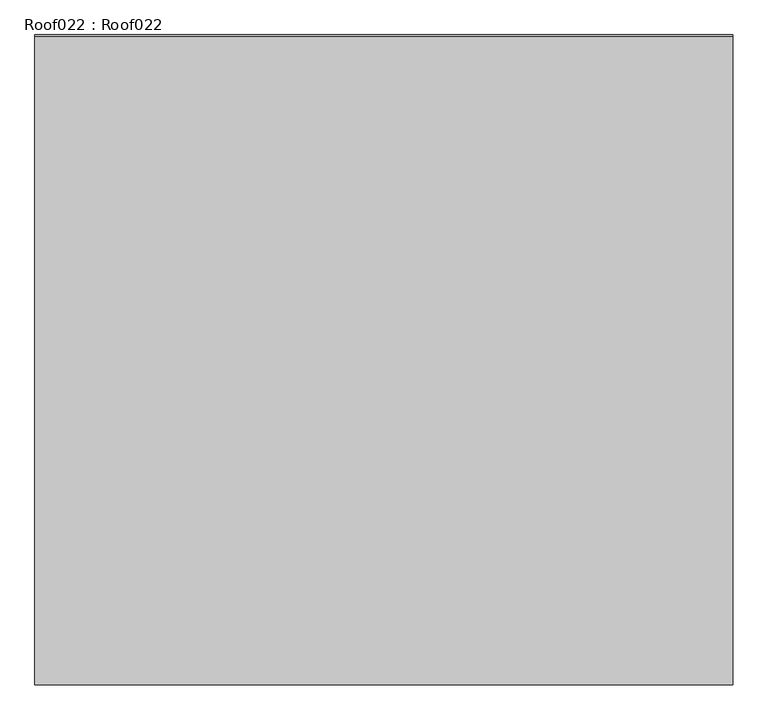
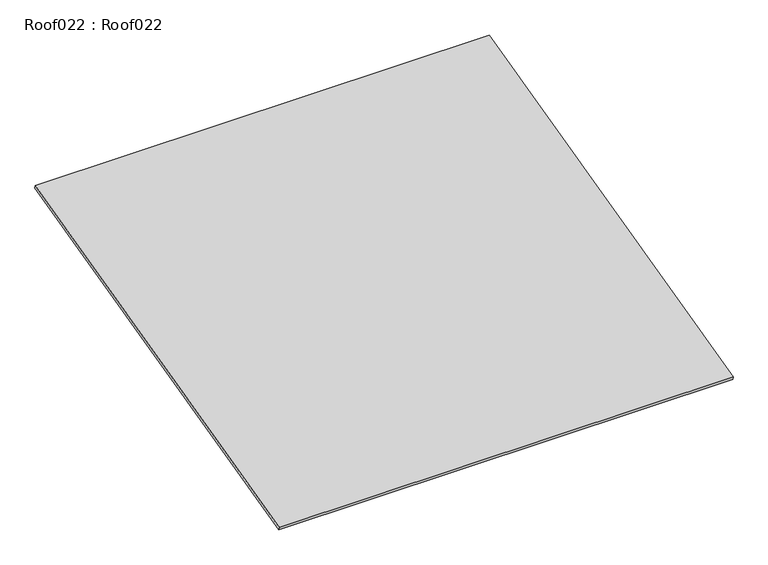
"""IFC4 building model written with IfcOpenShell, lengths in millimetres: proxy geometry, Roof022 : Roof022."""

from ifc_helpers import new_model, si_unit, frame, origin, place, context, project, spatial, polyline, outline, extrude, source, transform, mapped, element, save


def roof022_roof022_008d37f7(model_context):
    return source(origin(), model_context, "Body", "SweptSolid", [
        extrude(outline(polyline([(-5234.533266, 42865.9144838), (-3374.6402056, 43330.885847), (-3371.3378159, 43317.6762882), (-5231.2304687, 42852.703125), (-5234.533266, 42865.9144838)])), frame((12383.0175781, 0.0, 0.0), z_axis=(1.0, 0.0, 0.0), x_axis=(0.0, 1.0, 0.0)), (0.0, 0.0, 1.0), 2000.0),
    ])


if __name__ == "__main__":
    model = new_model("IFC4")
    model_context = context("Model", 3, world=origin())
    ifc_project = project(units=[si_unit("LENGTHUNIT", "METRE", prefix="MILLI")], contexts=[model_context])
    site = spatial("IfcSite", under=ifc_project)
    building = spatial("IfcBuilding", under=site)
    placement = place(None, origin())
    roof022_roof022_shape = roof022_roof022_008d37f7(model_context)
    element("IfcBuildingElementProxy", 1, Name="Roof022 : Roof022", ObjectType="Roof022 : Roof022", at=placement, inside=building, context=model_context, shape_type="MappedRepresentation", body=[
        mapped(roof022_roof022_shape, transform((0.0, 0.0, 0.0), x_axis=(1.0, 0.0, 0.0), y_axis=(0.0, 1.0, 0.0), z_axis=(0.0, 0.0, 1.0))),
    ])
    save(model, "model.ifc")

# Revit data of these elements
# Project information
#   Issued Date 1 = "0/00/2018 - City of Newport Beach"
#   IfcSite GUID = "26Pw6q$$GHwAGK093rt3ko"
#   IfcBuilding GUID = "26PxWq$$GHwAGK093rt3ko"
#   IfcProject GUID = "3580753c_1e44_4e66_87a"
#   NameOverride = "Default Site"
#   Project Issue Date = "Issue Date"
#   Project Status = "Project Status"
#   Client Name = "McElroy Residence"
#   Project Address = "New Single Family Residence (#010-2018)\n226 Tustin Ave,\nNewport Beach, CA 92663"
#   Project Name = "STAUDENMEIER RESIDENCE"
# Type "Roof022 : Roof022"
#   NameOverride = "Roof022"
# Element 1 (IfcBuildingElementProxy, "Roof022 : Roof022")
#   Materials on its faces: "STANDING SEAM METAL ROOF"
# Materials
#   "STANDING SEAM METAL ROOF": class "Unassigned", colour RGB 128 128 128, transparency 0
